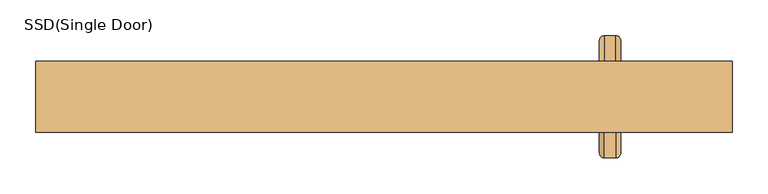
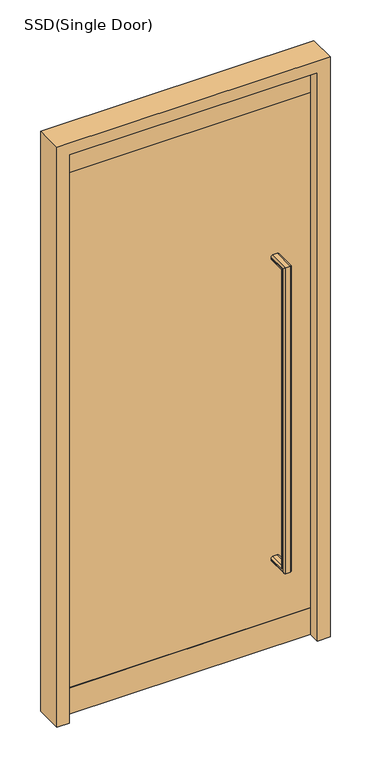
"""IFC4 building model written with IfcOpenShell, lengths in millimetres: door geometry, SSD(Single Door) : H_DR_AR B12_Door_Single_Glass_W1000xH2200_SSD-1."""

import ifcopenshell
import ifcopenshell.guid

model = None  # the IFC model being written
_history = None  # IfcOwnerHistory: only IFC2X3 demands one
_inside = {}  # id of a spatial element -> (the spatial element, [elements in it])
_under = {}  # id of a project, library or spatial element -> (it, [spatial elements below it])
_declared = {}  # id of a project -> (the project, [libraries it declares])
_typed = {}  # id of a type object -> (the type object, [elements of that type])
_made_of = {}  # id of a material, layer set ... -> (it, [elements and type objects made of it])


def new_model(schema):
    """Start an empty IFC model of exactly this schema.

    Asked for "IFC4X3", IfcOpenShell would pick the latest addendum, in which some entities
    have other attributes; the version numbers below select the first issue.
    IFC2X3 requires an IfcOwnerHistory on every rooted entity: one is made here for all.
    """
    global model, _history
    if schema == "IFC4X3":
        model = ifcopenshell.file(schema_version=(4, 3, 0, 0))
    else:
        model = ifcopenshell.file(schema=schema)
    _inside.clear()
    _under.clear()
    _declared.clear()
    _typed.clear()
    _made_of.clear()
    _history = None
    if model.schema == "IFC2X3":
        org = make("IfcOrganization", Name="unknown")
        user = make(
            "IfcPersonAndOrganization",
            ThePerson=make("IfcPerson", FamilyName="unknown"),
            TheOrganization=org,
        )
        app = make(
            "IfcApplication",
            ApplicationDeveloper=org,
            Version="unknown",
            ApplicationFullName="unknown",
            ApplicationIdentifier="unknown",
        )
        _history = make(
            "IfcOwnerHistory",
            OwningUser=user,
            OwningApplication=app,
            ChangeAction="ADDED",
            CreationDate=0,
        )
    return model


def make(cls, **values):
    """One entity of the class cls with the attributes given. An attribute that is None is left unset."""
    return model.create_entity(
        cls, **{name: value for name, value in values.items() if value is not None}
    )


def rooted(cls, **values):
    """An entity with a GlobalId (a new one), such as an element, a storey or a relation."""
    return make(cls, GlobalId=ifcopenshell.guid.new(), OwnerHistory=_history, **values)


def si_unit(unit_type, name, prefix=None):
    """IfcSIUnit, for example si_unit("LENGTHUNIT", "METRE", prefix="MILLI")."""
    return make("IfcSIUnit", UnitType=unit_type, Prefix=prefix, Name=name)


def assignment(units):
    """IfcUnitAssignment: the units of a project."""
    return None if units is None else make("IfcUnitAssignment", Units=units)


def point(xyz):
    """IfcCartesianPoint."""
    return None if xyz is None else make("IfcCartesianPoint", Coordinates=xyz)


def direction(xyz):
    """IfcDirection."""
    return None if xyz is None else make("IfcDirection", DirectionRatios=xyz)


def frame(location, z_axis=None, x_axis=None):
    """IfcAxis2Placement3D, a coordinate frame: its origin and axes. An axis left out is left unset."""
    return make(
        "IfcAxis2Placement3D",
        Location=point(location),
        Axis=direction(z_axis),
        RefDirection=direction(x_axis),
    )


def origin():
    """The frame at (0, 0, 0) with its axes left unset."""
    return frame((0.0, 0.0, 0.0))


def origin_with_axes():
    """The frame at (0, 0, 0) with the z axis (0, 0, 1) and the x axis (1, 0, 0) written out."""
    return frame((0.0, 0.0, 0.0), z_axis=(0.0, 0.0, 1.0), x_axis=(1.0, 0.0, 0.0))


def place(relative_to, where):
    """IfcLocalPlacement: puts the frame where relative to a parent placement (None: the world)."""
    return make(
        "IfcLocalPlacement", PlacementRelTo=relative_to, RelativePlacement=where
    )


def context(
    kind, dimensions, precision=None, world=None, true_north=None, identifier=None
):
    """IfcGeometricRepresentationContext, for example the 3D "Model" context."""
    return make(
        "IfcGeometricRepresentationContext",
        ContextIdentifier=identifier,
        ContextType=kind,
        CoordinateSpaceDimension=dimensions,
        Precision=precision,
        WorldCoordinateSystem=world,
        TrueNorth=true_north,
    )


def project(units=None, contexts=None):
    """IfcProject with its units and contexts."""
    return rooted(
        "IfcProject",
        Name="project",
        RepresentationContexts=contexts,
        UnitsInContext=assignment(units),
    )


def spatial(cls, under=None, at=None, **own):
    """A site, building, storey or space (cls), placed at a placement, below another one or the project."""
    s = rooted(cls, ObjectPlacement=at, **own)
    if under is not None:
        _under.setdefault(under.id(), (under, []))[1].append(s)
    return s


def polyline(points):
    """IfcPolyline through the points."""
    return make("IfcPolyline", Points=[point(p) for p in points])


def circle_curve(where, radius):
    """IfcCircle in the frame where."""
    return make("IfcCircle", Position=where, Radius=radius)


def ellipse_curve(where, semi_axis1, semi_axis2):
    """IfcEllipse in the frame where."""
    return make(
        "IfcEllipse", Position=where, SemiAxis1=semi_axis1, SemiAxis2=semi_axis2
    )


def outline(outer, holes=None, kind="AREA"):
    """IfcArbitraryClosedProfileDef: a profile drawn as a closed curve; with holes, ...WithVoids."""
    if holes is None:
        return make("IfcArbitraryClosedProfileDef", ProfileType=kind, OuterCurve=outer)
    return make(
        "IfcArbitraryProfileDefWithVoids",
        ProfileType=kind,
        OuterCurve=outer,
        InnerCurves=holes,
    )


def extrude(swept, where, along, depth):
    """IfcExtrudedAreaSolid: the profile swept, set in the frame where, extruded along a direction by depth."""
    return make(
        "IfcExtrudedAreaSolid",
        SweptArea=swept,
        Position=where,
        ExtrudedDirection=direction(along),
        Depth=depth,
    )


def shape(context_of_items, identifier, shape_type, items):
    """IfcShapeRepresentation: the items that make up one representation, for example the "Body"."""
    return make(
        "IfcShapeRepresentation",
        ContextOfItems=context_of_items,
        RepresentationIdentifier=identifier,
        RepresentationType=shape_type,
        Items=items,
    )


def source(mapping_origin, context_of_items, identifier, shape_type, items):
    """IfcRepresentationMap: a shape defined once, which mapped items show again and again."""
    return make(
        "IfcRepresentationMap",
        MappingOrigin=mapping_origin,
        MappedRepresentation=shape(context_of_items, identifier, shape_type, items),
    )


def transform(
    local_origin,
    x_axis=None,
    y_axis=None,
    z_axis=None,
    scale=None,
    scale2=None,
    scale3=None,
    uniform=True,
):
    """IfcCartesianTransformationOperator3D, or its non-uniform kind. x_axis, y_axis, z_axis: its Axis1, 2, 3."""
    if uniform:
        return make(
            "IfcCartesianTransformationOperator3D",
            Axis1=direction(x_axis),
            Axis2=direction(y_axis),
            LocalOrigin=point(local_origin),
            Scale=scale,
            Axis3=direction(z_axis),
        )
    return make(
        "IfcCartesianTransformationOperator3DnonUniform",
        Axis1=direction(x_axis),
        Axis2=direction(y_axis),
        LocalOrigin=point(local_origin),
        Scale=scale,
        Axis3=direction(z_axis),
        Scale2=scale2,
        Scale3=scale3,
    )


def mapped(mapping_source, mapping_target):
    """IfcMappedItem: shows the shape of a source again, moved by a transform."""
    return make(
        "IfcMappedItem", MappingSource=mapping_source, MappingTarget=mapping_target
    )


def made_of(thing, what):
    """Note that an element or type object is made of a material, layer set ...; save() writes the relation."""
    if what is not None:
        _made_of.setdefault(what.id(), (what, []))[1].append(thing)
    return thing


def element(
    cls,
    number,
    at=None,
    inside=None,
    cuts=None,
    type_object=None,
    material=None,
    context=None,
    identifier="Body",
    shape_type=None,
    held_by="IfcProductDefinitionShape",
    body=None,
    shapes=None,
    **own,
):
    """One element of the class cls, such as IfcWall. Its Tag is "e" and its number.

    at: its placement. inside: the storey or other place that contains it. cuts: it is an
    opening in that element (IfcRelVoidsElement). A single representation is given by context,
    identifier, shape_type and body (its items); several are given by shapes. held_by: the class
    of the entity that holds the representations. save() writes the other relations.
    """
    e = rooted(cls, Tag="e%d" % number, ObjectPlacement=at, **own)
    if body is not None:
        shapes = [shape(context, identifier, shape_type, body)]
    if shapes is not None:
        e.Representation = make(held_by, Representations=shapes)
    if inside is not None:
        _inside.setdefault(inside.id(), (inside, []))[1].append(e)
    if cuts is not None:
        rooted(
            "IfcRelVoidsElement", RelatingBuildingElement=cuts, RelatedOpeningElement=e
        )
    if type_object is not None:
        _typed.setdefault(type_object.id(), (type_object, []))[1].append(e)
    return made_of(e, material)


def aggregate(whole, parts):
    """IfcRelAggregates: a whole, such as a stair, and the parts it consists of."""
    return rooted("IfcRelAggregates", RelatingObject=whole, RelatedObjects=parts)


def save(model, path):
    """Write the relations noted so far, then the file.

    IfcRelAggregates (storeys below a building ...), IfcRelContainedInSpatialStructure (elements
    in a storey), IfcRelDefinesByType, IfcRelAssociatesMaterial and IfcRelDeclares: one each for
    every whole, place, type object, material and project.
    """
    for whole, parts in _under.values():
        aggregate(whole, parts)
    for where, things in _inside.values():
        rooted(
            "IfcRelContainedInSpatialStructure",
            RelatedElements=things,
            RelatingStructure=where,
        )
    for kind, things in _typed.values():
        rooted("IfcRelDefinesByType", RelatedObjects=things, RelatingType=kind)
    for what, things in _made_of.values():
        rooted("IfcRelAssociatesMaterial", RelatedObjects=things, RelatingMaterial=what)
    for by, libraries in _declared.values():
        rooted("IfcRelDeclares", RelatingContext=by, RelatedDefinitions=libraries)
    model.write(path)


def plane_surface(at):
    """IfcPlane: the flat surface through the origin of the frame at, square to its z axis."""
    return make("IfcPlane", Position=at)


def cylinder_surface(at, radius):
    """IfcCylindricalSurface: all points at the distance radius from the z axis of the frame at."""
    return make("IfcCylindricalSurface", Position=at, Radius=radius)


def advanced_brep(points, edges, surfaces, faces):
    """IfcAdvancedBrep: a solid bounded by faces that lie on surfaces and meet in shared edges.

    An edge is (start, end): straight between two places in points (the first is 0);
    or (start, end, curve); or (start, end, curve, False) where it runs against its curve.
    A face is (place in surfaces, loops), or (place, loops, False) where it looks against
    its surface's normal. A loop lists edges by number (the first is 1), with a minus sign
    where the edge is run from its end to its start. The first loop is the outer one.
    """
    corners = [point(p) for p in points]
    vertices = [make("IfcVertexPoint", VertexGeometry=c) for c in corners]
    made = []
    for start, end, *more in edges:
        made.append(
            make(
                "IfcEdgeCurve",
                EdgeStart=vertices[start],
                EdgeEnd=vertices[end],
                EdgeGeometry=more[0] if more else make("IfcPolyline", Points=[corners[start], corners[end]]),
                SameSense=more[1] if len(more) > 1 else True,
            )
        )
    hull = []
    for where, loops, *sense in faces:
        bounds = []
        for j, loop in enumerate(loops):
            ring = [make("IfcOrientedEdge", EdgeElement=made[abs(k) - 1], Orientation=k > 0) for k in loop]
            bounds.append(
                make(
                    "IfcFaceOuterBound" if j == 0 else "IfcFaceBound",
                    Bound=make("IfcEdgeLoop", EdgeList=ring),
                    Orientation=True,
                )
            )
        hull.append(make("IfcAdvancedFace", Bounds=bounds, FaceSurface=surfaces[where], SameSense=sense[0] if sense else True))
    return make("IfcAdvancedBrep", Outer=make("IfcClosedShell", CfsFaces=hull))


def ssd_single_door_d0e6de12(model_context):
    return source(origin(), model_context, "Body", "SolidModel", [
        extrude(outline(polyline([(0.0, -490.0), (0.0, -445.0), (2155.0, -445.0), (2155.0, 445.0), (0.0, 445.0), (0.0, 490.0), (2200.0, 490.0), (2200.0, -490.0), (0.0, -490.0)])), frame((0.0, 5.0, 0.0), z_axis=(0.0, 1.0, 0.0), x_axis=(0.0, 0.0, 1.0)), (0.0, 0.0, 1.0), 100.0),
        advanced_brep(
        [(310.0, 49.0, 1485.0), (326.0, 49.0, 1485.0), (333.0, 49.0, 1478.0), (333.0, 49.0, 1475.0), (326.0, 49.0, 1468.0), (310.0, 49.0, 1468.0), (303.0, 49.0, 1475.0), (303.0, 49.0, 1478.0), (310.0, 49.0, 325.0), (303.0, 49.0, 332.0), (303.0, 49.0, 335.0), (310.0, 49.0, 342.0), (326.0, 49.0, 342.0), (333.0, 49.0, 335.0), (333.0, 49.0, 332.0), (326.0, 49.0, 325.0), (310.0, -31.0, 1485.0), (326.0, -31.0, 1485.0), (333.0, -24.0, 1478.0), (333.0, -24.0, 332.0), (333.0, -21.0, 335.0), (333.0, -21.0, 1475.0), (326.0, -14.0, 1468.0), (310.0, -14.0, 1468.0), (303.0, -21.0, 1475.0), (303.0, -21.0, 335.0), (303.0, -24.0, 332.0), (303.0, -24.0, 1478.0), (310.0, -31.0, 325.0), (326.0, -31.0, 325.0), (326.0, -14.0, 342.0), (310.0, -14.0, 342.0)],
        [
            (0, 1),
            (1, 2, circle_curve(frame((326.0, 49.0, 1478.0), z_axis=(0.0, 1.0, 0.0), x_axis=(0.0, 0.0, -1.0)), 7.0)),
            (2, 3),
            (3, 4, circle_curve(frame((326.0, 49.0, 1475.0), z_axis=(0.0, 1.0, 0.0), x_axis=(0.0, 0.0, -1.0)), 7.0)),
            (4, 5),
            (5, 6, circle_curve(frame((310.0, 49.0, 1475.0), z_axis=(0.0, 1.0, 0.0), x_axis=(0.0, 0.0, -1.0)), 7.0)),
            (6, 7),
            (7, 0, circle_curve(frame((310.0, 49.0, 1478.0), z_axis=(0.0, 1.0, 0.0), x_axis=(0.0, 0.0, -1.0)), 7.0)),
            (8, 9, circle_curve(frame((310.0, 49.0, 332.0), z_axis=(0.0, 1.0, 0.0), x_axis=(0.0, 0.0, 1.0)), 7.0)),
            (9, 10),
            (10, 11, circle_curve(frame((310.0, 49.0, 335.0), z_axis=(0.0, 1.0, 0.0), x_axis=(0.0, 0.0, 1.0)), 7.0)),
            (11, 12),
            (12, 13, circle_curve(frame((326.0, 49.0, 335.0), z_axis=(0.0, 1.0, 0.0), x_axis=(0.0, 0.0, 1.0)), 7.0)),
            (13, 14),
            (14, 15, circle_curve(frame((326.0, 49.0, 332.0), z_axis=(0.0, 1.0, 0.0), x_axis=(0.0, 0.0, 1.0)), 7.0)),
            (15, 8),
            (0, 16),
            (16, 17),
            (17, 1),
            (17, 18, ellipse_curve(frame((326.0, -24.0, 1478.0), z_axis=(0.0, 0.7071067811865475, 0.7071067811865475), x_axis=(0.0, 0.7071067811865476, -0.7071067811865474)), 9.8994949, 7.0)),
            (18, 2),
            (18, 19),
            (19, 14),
            (13, 20),
            (20, 21),
            (21, 3),
            (21, 22, ellipse_curve(frame((326.0, -21.0, 1475.0), z_axis=(0.0, 0.7071067811865475, 0.7071067811865475), x_axis=(0.0, 0.7071067811865476, -0.7071067811865474)), 9.8994949, 7.0)),
            (22, 4),
            (22, 23),
            (23, 5),
            (23, 24, ellipse_curve(frame((310.0, -21.0, 1475.0), z_axis=(0.0, 0.7071067811865475, 0.7071067811865475), x_axis=(0.0, 0.7071067811865476, -0.7071067811865474)), 9.8994949, 7.0)),
            (24, 6),
            (24, 25),
            (25, 10),
            (9, 26),
            (26, 27),
            (27, 7),
            (27, 16, ellipse_curve(frame((310.0, -24.0, 1478.0), z_axis=(0.0, 0.7071067811865475, 0.7071067811865475), x_axis=(0.0, 0.7071067811865476, -0.7071067811865474)), 9.8994949, 7.0)),
            (16, 28),
            (28, 29),
            (29, 17),
            (29, 19, ellipse_curve(frame((326.0, -24.0, 332.0), z_axis=(0.0, -0.7071067811865475, 0.7071067811865475), x_axis=(0.0, 0.7071067811865474, 0.7071067811865476)), 9.8994949, 7.0)),
            (20, 30, ellipse_curve(frame((326.0, -21.0, 335.0), z_axis=(0.0, -0.7071067811865475, 0.7071067811865475), x_axis=(0.0, 0.7071067811865474, 0.7071067811865476)), 9.8994949, 7.0)),
            (30, 22),
            (30, 31),
            (31, 23),
            (31, 25, ellipse_curve(frame((310.0, -21.0, 335.0), z_axis=(0.0, -0.7071067811865475, 0.7071067811865475), x_axis=(0.0, 0.7071067811865474, 0.7071067811865476)), 9.8994949, 7.0)),
            (26, 28, ellipse_curve(frame((310.0, -24.0, 332.0), z_axis=(0.0, -0.7071067811865475, 0.7071067811865475), x_axis=(0.0, 0.7071067811865474, 0.7071067811865476)), 9.8994949, 7.0)),
            (28, 8),
            (15, 29),
            (12, 30),
            (11, 31),
        ],
        [
            plane_surface(frame((0.0, 49.0, 1485.0), z_axis=(0.0, 1.0, 0.0), x_axis=(1.0, 0.0, 0.0))),
            plane_surface(frame((0.0, 49.0, 325.0), z_axis=(0.0, 1.0, 0.0), x_axis=(1.0, 0.0, 0.0))),
            plane_surface(frame((310.0, 49.0, 1485.0), z_axis=(0.0, 0.0, 1.0), x_axis=(0.0, -1.0, 0.0))),
            cylinder_surface(frame((326.0, 49.0, 1478.0), z_axis=(0.0, 1.0, 0.0), x_axis=(0.0, 0.0, -1.0)), 7.0),
            plane_surface(frame((333.0, 49.0, 1478.0), z_axis=(1.0, 0.0, 0.0), x_axis=(0.0, -1.0, 0.0))),
            cylinder_surface(frame((326.0, 49.0, 1475.0), z_axis=(0.0, 1.0, 0.0), x_axis=(0.0, 0.0, -1.0)), 7.0),
            plane_surface(frame((326.0, 49.0, 1468.0), z_axis=(0.0, 0.0, -1.0), x_axis=(0.0, -1.0, 0.0))),
            cylinder_surface(frame((310.0, 49.0, 1475.0), z_axis=(0.0, 1.0, 0.0), x_axis=(0.0, 0.0, -1.0)), 7.0),
            plane_surface(frame((303.0, 49.0, 1475.0), z_axis=(-1.0, 0.0, 0.0), x_axis=(0.0, -1.0, 0.0))),
            cylinder_surface(frame((310.0, 49.0, 1478.0), z_axis=(0.0, 1.0, 0.0), x_axis=(0.0, 0.0, -1.0)), 7.0),
            plane_surface(frame((310.0, -31.0, 1485.0), z_axis=(0.0, -1.0, 0.0), x_axis=(0.0, 0.0, -1.0))),
            cylinder_surface(frame((326.0, -24.0, 1485.0), z_axis=(0.0, 0.0, 1.0), x_axis=(0.0, 1.0, 0.0)), 7.0),
            cylinder_surface(frame((326.0, -21.0, 1485.0), z_axis=(0.0, 0.0, 1.0), x_axis=(0.0, 1.0, 0.0)), 7.0),
            plane_surface(frame((326.0, -14.0, 1468.0), z_axis=(0.0, 1.0, 0.0), x_axis=(0.0, 0.0, -1.0))),
            cylinder_surface(frame((310.0, -21.0, 1485.0), z_axis=(0.0, 0.0, 1.0), x_axis=(0.0, 1.0, 0.0)), 7.0),
            cylinder_surface(frame((310.0, -24.0, 1485.0), z_axis=(0.0, 0.0, 1.0), x_axis=(0.0, 1.0, 0.0)), 7.0),
            plane_surface(frame((310.0, -31.0, 325.0), z_axis=(0.0, 0.0, -1.0), x_axis=(0.0, 1.0, 0.0))),
            cylinder_surface(frame((326.0, -31.0, 332.0), z_axis=(0.0, -1.0, 0.0), x_axis=(0.0, 0.0, 1.0)), 7.0),
            cylinder_surface(frame((326.0, -31.0, 335.0), z_axis=(0.0, -1.0, 0.0), x_axis=(0.0, 0.0, 1.0)), 7.0),
            plane_surface(frame((326.0, -14.0, 342.0), z_axis=(0.0, 0.0, 1.0), x_axis=(0.0, 1.0, 0.0))),
            cylinder_surface(frame((310.0, -31.0, 335.0), z_axis=(0.0, -1.0, 0.0), x_axis=(0.0, 0.0, 1.0)), 7.0),
            cylinder_surface(frame((310.0, -31.0, 332.0), z_axis=(0.0, -1.0, 0.0), x_axis=(0.0, 0.0, 1.0)), 7.0),
        ],
        [
            (0, [[1, 2, 3, 4, 5, 6, 7, 8]]),
            (1, [[9, 10, 11, 12, 13, 14, 15, 16]]),
            (2, [[-1, 17, 18, 19]]),
            (3, [[-2, -19, 20, 21]]),
            (4, [[-3, -21, 22, 23, -14, 24, 25, 26]]),
            (5, [[-4, -26, 27, 28]]),
            (6, [[-5, -28, 29, 30]]),
            (7, [[-6, -30, 31, 32]]),
            (8, [[-7, -32, 33, 34, -10, 35, 36, 37]]),
            (9, [[-8, -37, 38, -17]]),
            (10, [[-18, 39, 40, 41]]),
            (11, [[-20, -41, 42, -22]]),
            (12, [[-27, -25, 43, 44]]),
            (13, [[-29, -44, 45, 46]]),
            (14, [[-31, -46, 47, -33]]),
            (15, [[-38, -36, 48, -39]]),
            (16, [[-40, 49, -16, 50]]),
            (17, [[-42, -50, -15, -23]]),
            (18, [[-43, -24, -13, 51]]),
            (19, [[-45, -51, -12, 52]]),
            (20, [[-47, -52, -11, -34]]),
            (21, [[-48, -35, -9, -49]]),
        ],
    ),
        advanced_brep(
        [(310.0, 61.0, 1485.0), (303.0, 61.0, 1478.0), (303.0, 61.0, 1475.0), (310.0, 61.0, 1468.0), (326.0, 61.0, 1468.0), (333.0, 61.0, 1475.0), (333.0, 61.0, 1478.0), (326.0, 61.0, 1485.0), (310.0, 61.0, 325.0), (326.0, 61.0, 325.0), (333.0, 61.0, 332.0), (333.0, 61.0, 335.0), (326.0, 61.0, 342.0), (310.0, 61.0, 342.0), (303.0, 61.0, 335.0), (303.0, 61.0, 332.0), (310.0, 141.0, 1485.0), (303.0, 134.0, 1478.0), (303.0, 134.0, 332.0), (303.0, 131.0, 335.0), (303.0, 131.0, 1475.0), (310.0, 124.0, 1468.0), (326.0, 124.0, 1468.0), (333.0, 131.0, 1475.0), (333.0, 131.0, 335.0), (333.0, 134.0, 332.0), (333.0, 134.0, 1478.0), (326.0, 141.0, 1485.0), (310.0, 141.0, 325.0), (310.0, 124.0, 342.0), (326.0, 124.0, 342.0), (326.0, 141.0, 325.0)],
        [
            (0, 1, circle_curve(frame((310.0, 61.0, 1478.0), z_axis=(0.0, -1.0, 0.0), x_axis=(0.0, 0.0, 1.0)), 7.0)),
            (1, 2),
            (2, 3, circle_curve(frame((310.0, 61.0, 1475.0), z_axis=(0.0, -1.0, 0.0), x_axis=(0.0, 0.0, 1.0)), 7.0)),
            (3, 4),
            (4, 5, circle_curve(frame((326.0, 61.0, 1475.0), z_axis=(0.0, -1.0, 0.0), x_axis=(0.0, 0.0, 1.0)), 7.0)),
            (5, 6),
            (6, 7, circle_curve(frame((326.0, 61.0, 1478.0), z_axis=(0.0, -1.0, 0.0), x_axis=(0.0, 0.0, 1.0)), 7.0)),
            (7, 0),
            (8, 9),
            (9, 10, circle_curve(frame((326.0, 61.0, 332.0), z_axis=(0.0, -1.0, 0.0), x_axis=(0.0, 0.0, -1.0)), 7.0)),
            (10, 11),
            (11, 12, circle_curve(frame((326.0, 61.0, 335.0), z_axis=(0.0, -1.0, 0.0), x_axis=(0.0, 0.0, -1.0)), 7.0)),
            (12, 13),
            (13, 14, circle_curve(frame((310.0, 61.0, 335.0), z_axis=(0.0, -1.0, 0.0), x_axis=(0.0, 0.0, -1.0)), 7.0)),
            (14, 15),
            (15, 8, circle_curve(frame((310.0, 61.0, 332.0), z_axis=(0.0, -1.0, 0.0), x_axis=(0.0, 0.0, -1.0)), 7.0)),
            (0, 16),
            (16, 17, ellipse_curve(frame((310.0, 134.0, 1478.0), z_axis=(0.0, -0.7071067811865475, 0.7071067811865475), x_axis=(0.0, -0.7071067811865476, -0.7071067811865474)), 9.8994949, 7.0)),
            (17, 1),
            (17, 18),
            (18, 15),
            (14, 19),
            (19, 20),
            (20, 2),
            (20, 21, ellipse_curve(frame((310.0, 131.0, 1475.0), z_axis=(0.0, -0.7071067811865475, 0.7071067811865475), x_axis=(0.0, -0.7071067811865476, -0.7071067811865474)), 9.8994949, 7.0)),
            (21, 3),
            (21, 22),
            (22, 4),
            (22, 23, ellipse_curve(frame((326.0, 131.0, 1475.0), z_axis=(0.0, -0.7071067811865475, 0.7071067811865475), x_axis=(0.0, -0.7071067811865476, -0.7071067811865474)), 9.8994949, 7.0)),
            (23, 5),
            (23, 24),
            (24, 11),
            (10, 25),
            (25, 26),
            (26, 6),
            (26, 27, ellipse_curve(frame((326.0, 134.0, 1478.0), z_axis=(0.0, -0.7071067811865475, 0.7071067811865475), x_axis=(0.0, -0.7071067811865476, -0.7071067811865474)), 9.8994949, 7.0)),
            (27, 7),
            (27, 16),
            (16, 28),
            (28, 18, ellipse_curve(frame((310.0, 134.0, 332.0), z_axis=(0.0, 0.7071067811865475, 0.7071067811865475), x_axis=(0.0, -0.7071067811865474, 0.7071067811865476)), 9.8994949, 7.0)),
            (19, 29, ellipse_curve(frame((310.0, 131.0, 335.0), z_axis=(0.0, 0.7071067811865475, 0.7071067811865475), x_axis=(0.0, -0.7071067811865474, 0.7071067811865476)), 9.8994949, 7.0)),
            (29, 21),
            (29, 30),
            (30, 22),
            (30, 24, ellipse_curve(frame((326.0, 131.0, 335.0), z_axis=(0.0, 0.7071067811865475, 0.7071067811865475), x_axis=(0.0, -0.7071067811865474, 0.7071067811865476)), 9.8994949, 7.0)),
            (25, 31, ellipse_curve(frame((326.0, 134.0, 332.0), z_axis=(0.0, 0.7071067811865475, 0.7071067811865475), x_axis=(0.0, -0.7071067811865474, 0.7071067811865476)), 9.8994949, 7.0)),
            (31, 27),
            (31, 28),
            (28, 8),
            (13, 29),
            (12, 30),
            (9, 31),
        ],
        [
            plane_surface(frame((0.0, 61.0, 1485.0), z_axis=(0.0, -1.0, 0.0), x_axis=(1.0, 0.0, 0.0))),
            plane_surface(frame((0.0, 61.0, 325.0), z_axis=(0.0, -1.0, 0.0), x_axis=(1.0, 0.0, 0.0))),
            cylinder_surface(frame((310.0, 61.0, 1478.0), z_axis=(0.0, -1.0, 0.0), x_axis=(0.0, 0.0, 1.0)), 7.0),
            plane_surface(frame((303.0, 61.0, 1478.0), z_axis=(-1.0, 0.0, 0.0), x_axis=(0.0, 1.0, 0.0))),
            cylinder_surface(frame((310.0, 61.0, 1475.0), z_axis=(0.0, -1.0, 0.0), x_axis=(0.0, 0.0, 1.0)), 7.0),
            plane_surface(frame((310.0, 61.0, 1468.0), z_axis=(0.0, 0.0, -1.0), x_axis=(0.0, 1.0, 0.0))),
            cylinder_surface(frame((326.0, 61.0, 1475.0), z_axis=(0.0, -1.0, 0.0), x_axis=(0.0, 0.0, 1.0)), 7.0),
            plane_surface(frame((333.0, 61.0, 1475.0), z_axis=(1.0, 0.0, 0.0), x_axis=(0.0, 1.0, 0.0))),
            cylinder_surface(frame((326.0, 61.0, 1478.0), z_axis=(0.0, -1.0, 0.0), x_axis=(0.0, 0.0, 1.0)), 7.0),
            plane_surface(frame((326.0, 61.0, 1485.0), z_axis=(0.0, 0.0, 1.0), x_axis=(0.0, 1.0, 0.0))),
            cylinder_surface(frame((310.0, 134.0, 1485.0), z_axis=(0.0, 0.0, 1.0), x_axis=(0.0, 1.0, 0.0)), 7.0),
            cylinder_surface(frame((310.0, 131.0, 1485.0), z_axis=(0.0, 0.0, 1.0), x_axis=(0.0, 1.0, 0.0)), 7.0),
            plane_surface(frame((310.0, 124.0, 1468.0), z_axis=(0.0, -1.0, 0.0), x_axis=(0.0, 0.0, -1.0))),
            cylinder_surface(frame((326.0, 131.0, 1485.0), z_axis=(0.0, 0.0, 1.0), x_axis=(0.0, 1.0, 0.0)), 7.0),
            cylinder_surface(frame((326.0, 134.0, 1485.0), z_axis=(0.0, 0.0, 1.0), x_axis=(0.0, 1.0, 0.0)), 7.0),
            plane_surface(frame((326.0, 141.0, 1485.0), z_axis=(0.0, 1.0, 0.0), x_axis=(0.0, 0.0, -1.0))),
            cylinder_surface(frame((310.0, 141.0, 332.0), z_axis=(0.0, 1.0, 0.0), x_axis=(0.0, 0.0, -1.0)), 7.0),
            cylinder_surface(frame((310.0, 141.0, 335.0), z_axis=(0.0, 1.0, 0.0), x_axis=(0.0, 0.0, -1.0)), 7.0),
            plane_surface(frame((310.0, 124.0, 342.0), z_axis=(0.0, 0.0, 1.0), x_axis=(0.0, -1.0, 0.0))),
            cylinder_surface(frame((326.0, 141.0, 335.0), z_axis=(0.0, 1.0, 0.0), x_axis=(0.0, 0.0, -1.0)), 7.0),
            cylinder_surface(frame((326.0, 141.0, 332.0), z_axis=(0.0, 1.0, 0.0), x_axis=(0.0, 0.0, -1.0)), 7.0),
            plane_surface(frame((326.0, 141.0, 325.0), z_axis=(0.0, 0.0, -1.0), x_axis=(0.0, -1.0, 0.0))),
        ],
        [
            (0, [[1, 2, 3, 4, 5, 6, 7, 8]]),
            (1, [[9, 10, 11, 12, 13, 14, 15, 16]]),
            (2, [[-1, 17, 18, 19]]),
            (3, [[-2, -19, 20, 21, -15, 22, 23, 24]]),
            (4, [[-3, -24, 25, 26]]),
            (5, [[-4, -26, 27, 28]]),
            (6, [[-5, -28, 29, 30]]),
            (7, [[-6, -30, 31, 32, -11, 33, 34, 35]]),
            (8, [[-7, -35, 36, 37]]),
            (9, [[-8, -37, 38, -17]]),
            (10, [[-18, 39, 40, -20]]),
            (11, [[-25, -23, 41, 42]]),
            (12, [[-27, -42, 43, 44]]),
            (13, [[-29, -44, 45, -31]]),
            (14, [[-36, -34, 46, 47]]),
            (15, [[-38, -47, 48, -39]]),
            (16, [[-40, 49, -16, -21]]),
            (17, [[-41, -22, -14, 50]]),
            (18, [[-43, -50, -13, 51]]),
            (19, [[-45, -51, -12, -32]]),
            (20, [[-46, -33, -10, 52]]),
            (21, [[-48, -52, -9, -49]]),
        ],
    ),
        extrude(outline(polyline([(445.0, 49.0), (-445.0, 49.0), (-445.0, 61.0), (445.0, 61.0), (445.0, 49.0)])), frame((0.0, 0.0, 100.0), z_axis=(0.0, 0.0, 1.0), x_axis=(1.0, 0.0, 0.0)), (0.0, 0.0, 1.0), 1955.0),
        extrude(outline(polyline([(445.0, 47.0), (-445.0, 47.0), (-445.0, 63.0), (445.0, 63.0), (445.0, 47.0)])), frame((0.0, 0.0, 2055.0), z_axis=(0.0, 0.0, 1.0), x_axis=(1.0, 0.0, 0.0)), (0.0, 0.0, 1.0), 100.0),
        extrude(outline(polyline([(445.0, 47.0), (-445.0, 47.0), (-445.0, 63.0), (445.0, 63.0), (445.0, 47.0)])), origin_with_axes(), (0.0, 0.0, 1.0), 100.0),
    ])


if __name__ == "__main__":
    model = new_model("IFC4")
    model_context = context("Model", 3, world=origin())
    ifc_project = project(units=[si_unit("LENGTHUNIT", "METRE", prefix="MILLI")], contexts=[model_context])
    site = spatial("IfcSite", under=ifc_project)
    building = spatial("IfcBuilding", under=site)
    placement = place(None, origin())
    ssd_single_door_shape = ssd_single_door_d0e6de12(model_context)
    element("IfcDoor", 1, ObjectType="SSD(Single Door) : H_DR_AR B12_Door_Single_Glass_W1000xH2200_SSD-1", at=placement, inside=building, context=model_context, shape_type="MappedRepresentation", body=[
        mapped(ssd_single_door_shape, transform((0.0, 0.0, 0.0), x_axis=(1.0, 0.0, 0.0), y_axis=(0.0, 1.0, 0.0), z_axis=(0.0, 0.0, 1.0))),
    ])
    save(model, "model.ifc")

# Revit data of these elements
# Type "SSD(Single Door) : H_DR_AR B12_Door_Single_Glass_W1000xH2200_SSD-1"
#   Type Mark = "452"
#   Type Comments = "SSD"
#   Analytic Construction = "<None>"
#   Thickness = 45 mm
#   Plan Door Swing2 = 890 mm
#   Plan Door Swing = 1780 mm
#   Glass Thk = 12 mm
#   Frame THK = 100 mm
#   Frame Projection Ext. = 25 mm
#   Frame Projection Int. = 25 mm
#   Frame Width = 75 mm
#   Height = 2200 mm
#   Width = 980 mm
#   Center Door [instance default] = 100 mm
#   Define Thermal Properties by = 1
#   Function = (empty or 0)
#   Wall Closure = (empty or 0)
# Element 1 (IfcDoor, "SSD(Single Door) : H_DR_AR B12_Door_Single_Glass_W1000xH2200_SSD-1")
#   Center Door = 55 mm
#   Materials on its faces: "Stainless Steel", "Glass"
# Materials
#   "Stainless Steel": class "Metal", colour RGB 189 187 185, transparency 0, Description = "Stainless Steel 18/8", Cost = 0
#   "Glass": class "Glass", colour RGB 218 227 224, transparency 0.85, Description = "Soda Lime Glass", Cost = 0
